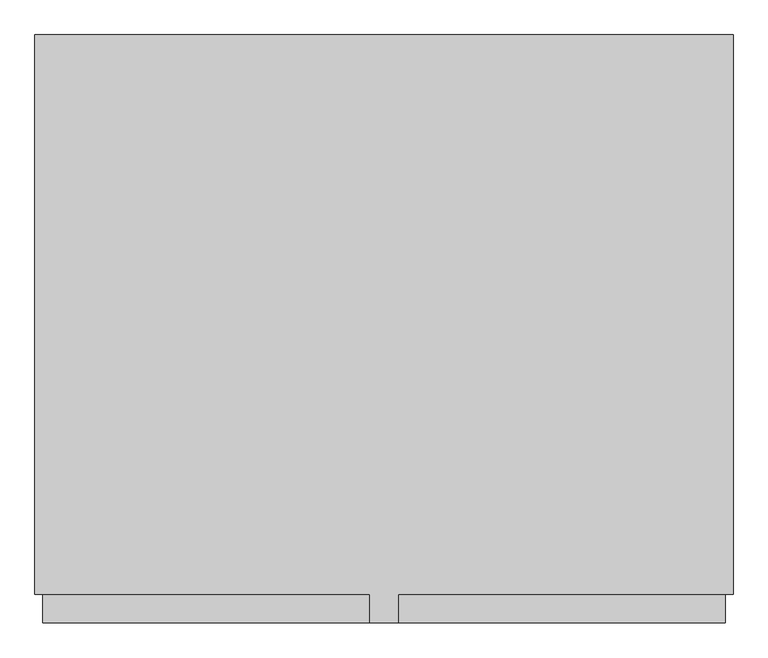
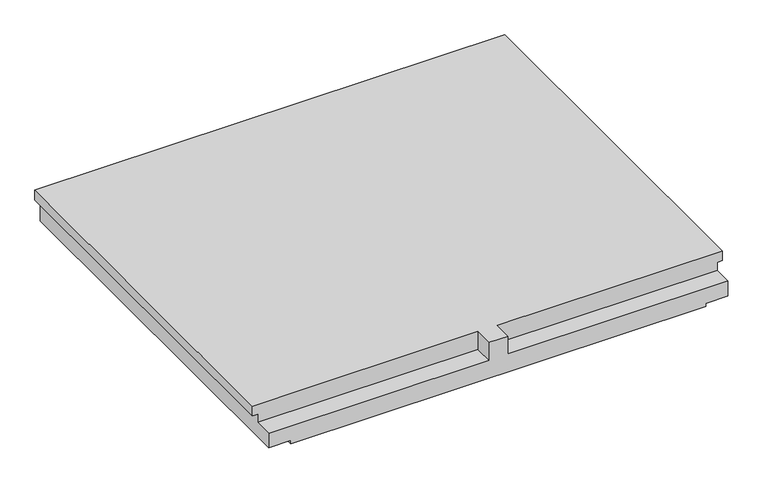
"""IFC4 building model written with IfcOpenShell, lengths in millimetres: stair geometry, NLRS_24_GM_UN_rechthoekig bordes prefab-AV_gen_rsf : prefab bordes_gen__2300x2730."""

from ifc_helpers import new_model, si_unit, origin, place, context, project, spatial, faceted_brep, source, transform, mapped, element, save


def stair_c7907445(model_context):
    return source(origin(), model_context, "Body", "Brep", [
        faceted_brep([(1365.0, -2190.0, 0.0), (1365.0, -2190.0, -60.0), (1365.0, 0.0, -60.0), (1365.0, 0.0, 0.0), (55.0, -2300.0, -110.0), (1335.0, -2300.0, -110.0), (1335.0, -2190.0, -110.0), (55.0, -2190.0, -110.0), (55.0, -2190.0, 0.0), (1335.0, -2190.0, -60.0), (55.0, -2300.0, 0.0), (-55.0, -2300.0, 0.0), (-55.0, -2190.0, 0.0), (-55.0, -2190.0, -110.0), (-55.0, -2300.0, -110.0), (-1365.0, 0.0, 0.0), (-1365.0, 0.0, -60.0), (-1365.0, -2190.0, -60.0), (-1365.0, -2190.0, 0.0), (-1335.0, -2300.0, -110.0), (-1335.0, -2300.0, -200.0), (-1205.0, -2300.0, -200.0), (-1205.0, -2300.0, -220.0), (1205.0, -2300.0, -220.0), (1205.0, -2300.0, -200.0), (1335.0, -2300.0, -200.0), (-1335.0, -2190.0, -110.0), (-1335.0, -2190.0, -60.0), (1335.0, 0.0, -60.0), (1335.0, 0.0, -200.0), (1205.0, 0.0, -200.0), (1205.0, 0.0, -220.0), (-1205.0, 0.0, -220.0), (-1205.0, 0.0, -200.0), (-1335.0, 0.0, -200.0), (-1335.0, 0.0, -60.0)], [[[0, 1, 2, 3]], [[4, 5, 6, 7]], [[8, 7, 6, 9, 1, 0]], [[10, 4, 7, 8]], [[11, 12, 13, 14]], [[15, 16, 17, 18]], [[19, 20, 21, 22, 23, 24, 25, 5, 4, 10, 11, 14]], [[14, 13, 26, 19]], [[18, 17, 27, 26, 13, 12]], [[18, 12, 11, 10, 8, 0, 3, 15]], [[15, 3, 2, 28, 29, 30, 31, 32, 33, 34, 35, 16]], [[32, 31, 23, 22]], [[27, 17, 16, 35]], [[20, 19, 26, 27, 35, 34]], [[34, 33, 21, 20]], [[33, 32, 22, 21]], [[28, 2, 1, 9]], [[29, 28, 9, 6, 5, 25]], [[25, 24, 30, 29]], [[24, 23, 31, 30]]]),
    ])


if __name__ == "__main__":
    model = new_model("IFC4")
    model_context = context("Model", 3, world=origin())
    ifc_project = project(units=[si_unit("LENGTHUNIT", "METRE", prefix="MILLI")], contexts=[model_context])
    site = spatial("IfcSite", under=ifc_project)
    building = spatial("IfcBuilding", under=site)
    placement = place(None, origin())
    stair_shape = stair_c7907445(model_context)
    element("IfcStair", 1, ObjectType="NLRS_24_GM_UN_rechthoekig bordes prefab-AV_gen_rsf : prefab bordes_gen__2300x2730", at=placement, inside=building, context=model_context, shape_type="MappedRepresentation", body=[
        mapped(stair_shape, transform((0.0, 0.0, 0.0), x_axis=(1.0, 0.0, 0.0), y_axis=(0.0, 1.0, 0.0), z_axis=(0.0, 0.0, 1.0))),
    ])
    save(model, "model.ifc")

# Revit data of these elements
# Type "NLRS_24_GM_UN_rechthoekig bordes prefab-AV_gen_rsf : prefab bordes_gen__2300x2730"
#   IfcExportAs = "IfcStair"
#   Type Comments = " "
#   Model = " "
#   Manufacturer = " "
#   Description = "rechthoekig bordes prefab\r\n1930x4395"
#   Assembly Code = "24.15"
#   Width = 2730 mm
#   Thickness = 220 mm
#   Perimeter = 10060 mm
#   NLRS_C_lengte_02 = 1310 mm
#   NLRS_C_lengte_01 = 1310 mm
#   NLRS_C_hoogte_02 = 110 mm
#   NLRS_C_hoogte_01 = 110 mm
#   NLRS_C_diepte_04 = 2300 mm
#   NLRS_C_diepte_03 = 2300 mm
#   NLRS_C_diepte_02 = 110 mm
#   NLRS_C_diepte_01 = 110 mm
#   Length = 2300 mm
#   Default Elevation = 1219.2 mm
#   Area = 6.279 m²
#   NLRS_C_materiaal = NLRS_f2_beton prefab_gen_rsf
#   Keynote = ""
# Element 1 (IfcStair, "NLRS_24_GM_UN_rechthoekig bordes prefab-AV_gen_rsf : prefab bordes_gen__2300x2730")
#   Materials on its faces: "NLRS_f2_beton prefab_gen_rsf"
# Materials
#   "NLRS_f2_beton prefab_gen_rsf": class "F - Niet gebakken kunststeen", colour RGB 129 133 118, transparency 0, Keynote = "f2", Manufacturer = "Revit Standards Foundation", URL = "www.revitstandards.org", Description = "beton prefab", Cost = 0
